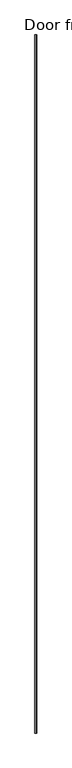
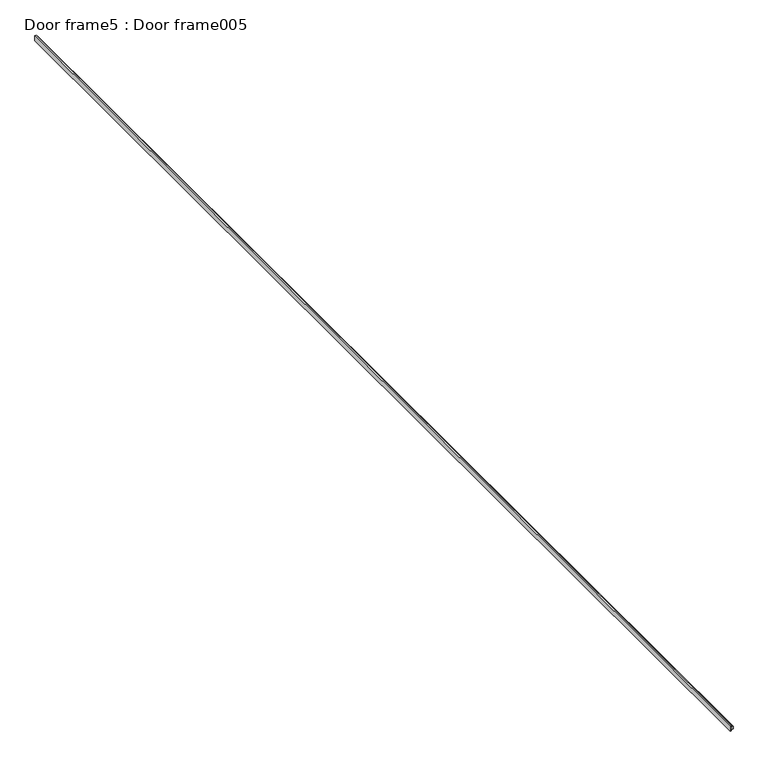
"""IFC4 building model written with IfcOpenShell, lengths in millimetres: proxy geometry, Door frame5 : Door frame005."""

from ifc_helpers import new_model, si_unit, frame, origin, place, context, project, spatial, polyline, outline, extrude, source, transform, mapped, element, save


def door_frame5_door_frame005_abb10e86(model_context):
    return source(origin(), model_context, "Body", "SweptSolid", [
        extrude(outline(polyline([(36678.7014343, 15555.3292246), (36678.7014343, 15557.5465976), (36682.2000947, 15557.5465976), (36682.2000947, 15559.3245976), (36680.8030947, 15559.3245976), (36680.8030947, 15560.3913976), (36685.3750947, 15560.3913976), (36685.3750947, 15559.3245976), (36683.9780947, 15559.3245976), (36683.9780947, 15557.546547), (36687.4772673, 15557.546547), (36687.4772673, 15555.3292246), (36678.7014343, 15555.3292246)])), frame((0.0, -1052.8906567, 0.0), z_axis=(0.0, 1.0, 0.0), x_axis=(0.0, 0.0, 1.0)), (0.0, 0.0, 1.0), 1999.85),
    ])


if __name__ == "__main__":
    model = new_model("IFC4")
    model_context = context("Model", 3, world=origin())
    ifc_project = project(units=[si_unit("LENGTHUNIT", "METRE", prefix="MILLI")], contexts=[model_context])
    site = spatial("IfcSite", under=ifc_project)
    building = spatial("IfcBuilding", under=site)
    placement = place(None, origin())
    door_frame5_door_frame005_shape = door_frame5_door_frame005_abb10e86(model_context)
    element("IfcBuildingElementProxy", 1, Name="Door frame5 : Door frame005", ObjectType="Door frame5 : Door frame005", at=placement, inside=building, context=model_context, shape_type="MappedRepresentation", body=[
        mapped(door_frame5_door_frame005_shape, transform((0.0, 0.0, 0.0), x_axis=(1.0, 0.0, 0.0), y_axis=(0.0, 1.0, 0.0), z_axis=(0.0, 0.0, 1.0))),
    ])
    save(model, "model.ifc")

# Revit data of these elements
# Type "Door frame5 : Door frame005"
#   NameOverride = "Door frame005"
# Element 1 (IfcBuildingElementProxy, "Door frame5 : Door frame005")
#   Materials on its faces: "FLEETWOOD SERIES T-3200 SINGLE SWING DOOR FRAME"
# Materials
#   "FLEETWOOD SERIES T-3200 SINGLE SWING DOOR FRAME": class "Unassigned", colour RGB 128 128 128, transparency 0, Cost = 0
